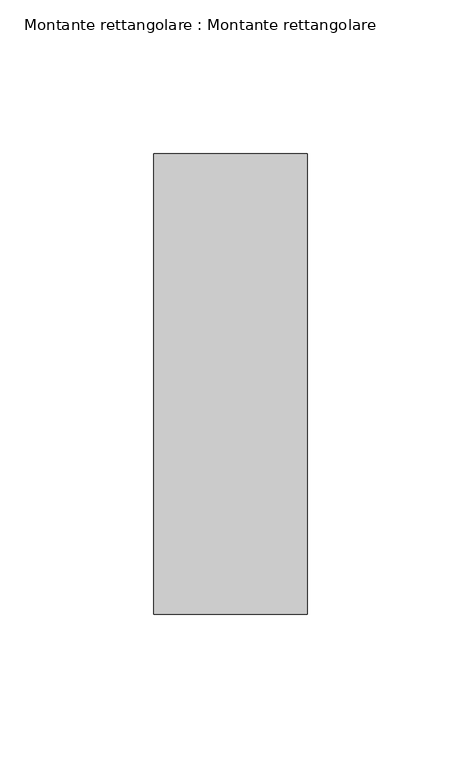
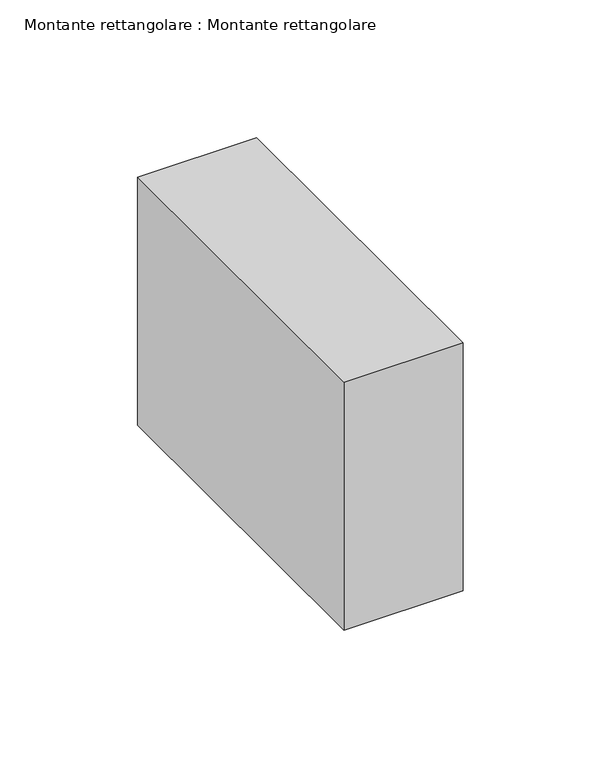
"""IFC4 building model written with IfcOpenShell, lengths in millimetres: member geometry, Montante rettangolare : Montante rettangolare."""

import ifcopenshell
import ifcopenshell.guid

model = None  # the IFC model being written
_history = None  # IfcOwnerHistory: only IFC2X3 demands one
_inside = {}  # id of a spatial element -> (the spatial element, [elements in it])
_under = {}  # id of a project, library or spatial element -> (it, [spatial elements below it])
_declared = {}  # id of a project -> (the project, [libraries it declares])
_typed = {}  # id of a type object -> (the type object, [elements of that type])
_made_of = {}  # id of a material, layer set ... -> (it, [elements and type objects made of it])


def new_model(schema):
    """Start an empty IFC model of exactly this schema.

    Asked for "IFC4X3", IfcOpenShell would pick the latest addendum, in which some entities
    have other attributes; the version numbers below select the first issue.
    IFC2X3 requires an IfcOwnerHistory on every rooted entity: one is made here for all.
    """
    global model, _history
    if schema == "IFC4X3":
        model = ifcopenshell.file(schema_version=(4, 3, 0, 0))
    else:
        model = ifcopenshell.file(schema=schema)
    _inside.clear()
    _under.clear()
    _declared.clear()
    _typed.clear()
    _made_of.clear()
    _history = None
    if model.schema == "IFC2X3":
        org = make("IfcOrganization", Name="unknown")
        user = make(
            "IfcPersonAndOrganization",
            ThePerson=make("IfcPerson", FamilyName="unknown"),
            TheOrganization=org,
        )
        app = make(
            "IfcApplication",
            ApplicationDeveloper=org,
            Version="unknown",
            ApplicationFullName="unknown",
            ApplicationIdentifier="unknown",
        )
        _history = make(
            "IfcOwnerHistory",
            OwningUser=user,
            OwningApplication=app,
            ChangeAction="ADDED",
            CreationDate=0,
        )
    return model


def make(cls, **values):
    """One entity of the class cls with the attributes given. An attribute that is None is left unset."""
    return model.create_entity(
        cls, **{name: value for name, value in values.items() if value is not None}
    )


def rooted(cls, **values):
    """An entity with a GlobalId (a new one), such as an element, a storey or a relation."""
    return make(cls, GlobalId=ifcopenshell.guid.new(), OwnerHistory=_history, **values)


def si_unit(unit_type, name, prefix=None):
    """IfcSIUnit, for example si_unit("LENGTHUNIT", "METRE", prefix="MILLI")."""
    return make("IfcSIUnit", UnitType=unit_type, Prefix=prefix, Name=name)


def assignment(units):
    """IfcUnitAssignment: the units of a project."""
    return None if units is None else make("IfcUnitAssignment", Units=units)


def point(xyz):
    """IfcCartesianPoint."""
    return None if xyz is None else make("IfcCartesianPoint", Coordinates=xyz)


def direction(xyz):
    """IfcDirection."""
    return None if xyz is None else make("IfcDirection", DirectionRatios=xyz)


def frame(location, z_axis=None, x_axis=None):
    """IfcAxis2Placement3D, a coordinate frame: its origin and axes. An axis left out is left unset."""
    return make(
        "IfcAxis2Placement3D",
        Location=point(location),
        Axis=direction(z_axis),
        RefDirection=direction(x_axis),
    )


def origin():
    """The frame at (0, 0, 0) with its axes left unset."""
    return frame((0.0, 0.0, 0.0))


def place(relative_to, where):
    """IfcLocalPlacement: puts the frame where relative to a parent placement (None: the world)."""
    return make(
        "IfcLocalPlacement", PlacementRelTo=relative_to, RelativePlacement=where
    )


def context(
    kind, dimensions, precision=None, world=None, true_north=None, identifier=None
):
    """IfcGeometricRepresentationContext, for example the 3D "Model" context."""
    return make(
        "IfcGeometricRepresentationContext",
        ContextIdentifier=identifier,
        ContextType=kind,
        CoordinateSpaceDimension=dimensions,
        Precision=precision,
        WorldCoordinateSystem=world,
        TrueNorth=true_north,
    )


def project(units=None, contexts=None):
    """IfcProject with its units and contexts."""
    return rooted(
        "IfcProject",
        Name="project",
        RepresentationContexts=contexts,
        UnitsInContext=assignment(units),
    )


def spatial(cls, under=None, at=None, **own):
    """A site, building, storey or space (cls), placed at a placement, below another one or the project."""
    s = rooted(cls, ObjectPlacement=at, **own)
    if under is not None:
        _under.setdefault(under.id(), (under, []))[1].append(s)
    return s


def polyline(points):
    """IfcPolyline through the points."""
    return make("IfcPolyline", Points=[point(p) for p in points])


def outline(outer, holes=None, kind="AREA"):
    """IfcArbitraryClosedProfileDef: a profile drawn as a closed curve; with holes, ...WithVoids."""
    if holes is None:
        return make("IfcArbitraryClosedProfileDef", ProfileType=kind, OuterCurve=outer)
    return make(
        "IfcArbitraryProfileDefWithVoids",
        ProfileType=kind,
        OuterCurve=outer,
        InnerCurves=holes,
    )


def extrude(swept, where, along, depth):
    """IfcExtrudedAreaSolid: the profile swept, set in the frame where, extruded along a direction by depth."""
    return make(
        "IfcExtrudedAreaSolid",
        SweptArea=swept,
        Position=where,
        ExtrudedDirection=direction(along),
        Depth=depth,
    )


def shape(context_of_items, identifier, shape_type, items):
    """IfcShapeRepresentation: the items that make up one representation, for example the "Body"."""
    return make(
        "IfcShapeRepresentation",
        ContextOfItems=context_of_items,
        RepresentationIdentifier=identifier,
        RepresentationType=shape_type,
        Items=items,
    )


def source(mapping_origin, context_of_items, identifier, shape_type, items):
    """IfcRepresentationMap: a shape defined once, which mapped items show again and again."""
    return make(
        "IfcRepresentationMap",
        MappingOrigin=mapping_origin,
        MappedRepresentation=shape(context_of_items, identifier, shape_type, items),
    )


def transform(
    local_origin,
    x_axis=None,
    y_axis=None,
    z_axis=None,
    scale=None,
    scale2=None,
    scale3=None,
    uniform=True,
):
    """IfcCartesianTransformationOperator3D, or its non-uniform kind. x_axis, y_axis, z_axis: its Axis1, 2, 3."""
    if uniform:
        return make(
            "IfcCartesianTransformationOperator3D",
            Axis1=direction(x_axis),
            Axis2=direction(y_axis),
            LocalOrigin=point(local_origin),
            Scale=scale,
            Axis3=direction(z_axis),
        )
    return make(
        "IfcCartesianTransformationOperator3DnonUniform",
        Axis1=direction(x_axis),
        Axis2=direction(y_axis),
        LocalOrigin=point(local_origin),
        Scale=scale,
        Axis3=direction(z_axis),
        Scale2=scale2,
        Scale3=scale3,
    )


def mapped(mapping_source, mapping_target):
    """IfcMappedItem: shows the shape of a source again, moved by a transform."""
    return make(
        "IfcMappedItem", MappingSource=mapping_source, MappingTarget=mapping_target
    )


def made_of(thing, what):
    """Note that an element or type object is made of a material, layer set ...; save() writes the relation."""
    if what is not None:
        _made_of.setdefault(what.id(), (what, []))[1].append(thing)
    return thing


def element(
    cls,
    number,
    at=None,
    inside=None,
    cuts=None,
    type_object=None,
    material=None,
    context=None,
    identifier="Body",
    shape_type=None,
    held_by="IfcProductDefinitionShape",
    body=None,
    shapes=None,
    **own,
):
    """One element of the class cls, such as IfcWall. Its Tag is "e" and its number.

    at: its placement. inside: the storey or other place that contains it. cuts: it is an
    opening in that element (IfcRelVoidsElement). A single representation is given by context,
    identifier, shape_type and body (its items); several are given by shapes. held_by: the class
    of the entity that holds the representations. save() writes the other relations.
    """
    e = rooted(cls, Tag="e%d" % number, ObjectPlacement=at, **own)
    if body is not None:
        shapes = [shape(context, identifier, shape_type, body)]
    if shapes is not None:
        e.Representation = make(held_by, Representations=shapes)
    if inside is not None:
        _inside.setdefault(inside.id(), (inside, []))[1].append(e)
    if cuts is not None:
        rooted(
            "IfcRelVoidsElement", RelatingBuildingElement=cuts, RelatedOpeningElement=e
        )
    if type_object is not None:
        _typed.setdefault(type_object.id(), (type_object, []))[1].append(e)
    return made_of(e, material)


def aggregate(whole, parts):
    """IfcRelAggregates: a whole, such as a stair, and the parts it consists of."""
    return rooted("IfcRelAggregates", RelatingObject=whole, RelatedObjects=parts)


def save(model, path):
    """Write the relations noted so far, then the file.

    IfcRelAggregates (storeys below a building ...), IfcRelContainedInSpatialStructure (elements
    in a storey), IfcRelDefinesByType, IfcRelAssociatesMaterial and IfcRelDeclares: one each for
    every whole, place, type object, material and project.
    """
    for whole, parts in _under.values():
        aggregate(whole, parts)
    for where, things in _inside.values():
        rooted(
            "IfcRelContainedInSpatialStructure",
            RelatedElements=things,
            RelatingStructure=where,
        )
    for kind, things in _typed.values():
        rooted("IfcRelDefinesByType", RelatedObjects=things, RelatingType=kind)
    for what, things in _made_of.values():
        rooted("IfcRelAssociatesMaterial", RelatedObjects=things, RelatingMaterial=what)
    for by, libraries in _declared.values():
        rooted("IfcRelDeclares", RelatingContext=by, RelatedDefinitions=libraries)
    model.write(path)


def montante_rettangolare_montante_rettangolare_fd833763(model_context):
    return source(origin(), model_context, "Body", "SweptSolid", [
        extrude(outline(polyline([(25.0, 75.0), (25.0, -75.0), (-25.0, -75.0), (-25.0, 75.0), (25.0, 75.0)])), frame((0.0, 0.0, -110.0), z_axis=(0.0, 0.0, 1.0), x_axis=(1.0, 0.0, 0.0)), (0.0, 0.0, 1.0), 110.0),
    ])


if __name__ == "__main__":
    model = new_model("IFC4")
    model_context = context("Model", 3, world=origin())
    ifc_project = project(units=[si_unit("LENGTHUNIT", "METRE", prefix="MILLI")], contexts=[model_context])
    site = spatial("IfcSite", under=ifc_project)
    building = spatial("IfcBuilding", under=site)
    placement = place(None, origin())
    montante_rettangolare_montante_rettangolare_shape = montante_rettangolare_montante_rettangolare_fd833763(model_context)
    element("IfcMember", 1, ObjectType="Montante rettangolare : Montante rettangolare", at=placement, inside=building, context=model_context, shape_type="MappedRepresentation", body=[
        mapped(montante_rettangolare_montante_rettangolare_shape, transform((0.0, 0.0, 0.0), x_axis=(1.0, 0.0, 0.0), y_axis=(0.0, 1.0, 0.0), z_axis=(0.0, 0.0, 1.0))),
    ])
    save(model, "model.ifc")

# Revit data of these elements
# Type "Montante rettangolare : Montante rettangolare"
#   built-in parameter 1007304 = 0.492126 (stored number, unit not read)
#   built-in parameter 1007301 = 0.082021 (stored number, unit not read)
#   built-in parameter 1007300 = 0.082021 (stored number, unit not read)
# Element 1 (IfcMember, "Montante rettangolare : Montante rettangolare")
#   Materials on its faces: "Acciaio"
# Materials
#   "Acciaio": class "Metallo", colour RGB 247 247 247, transparency 0, Description = "Acciaio, finitura zigrinata", Cost = 0
